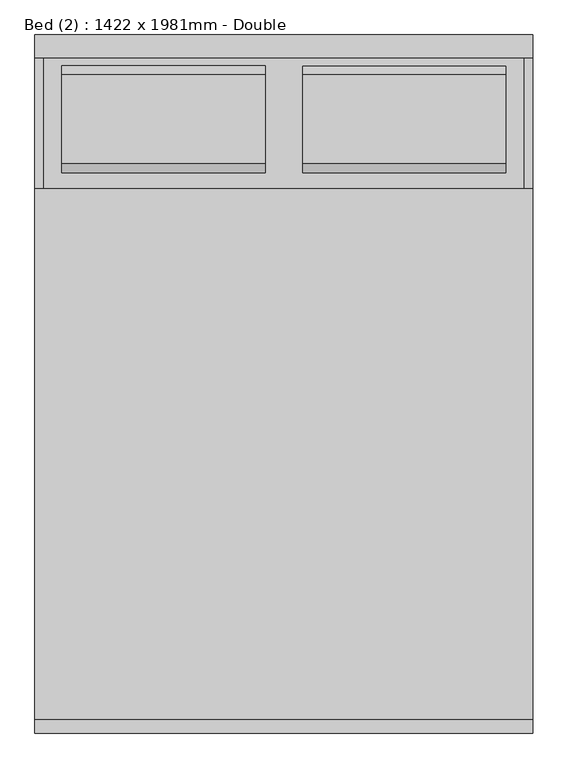
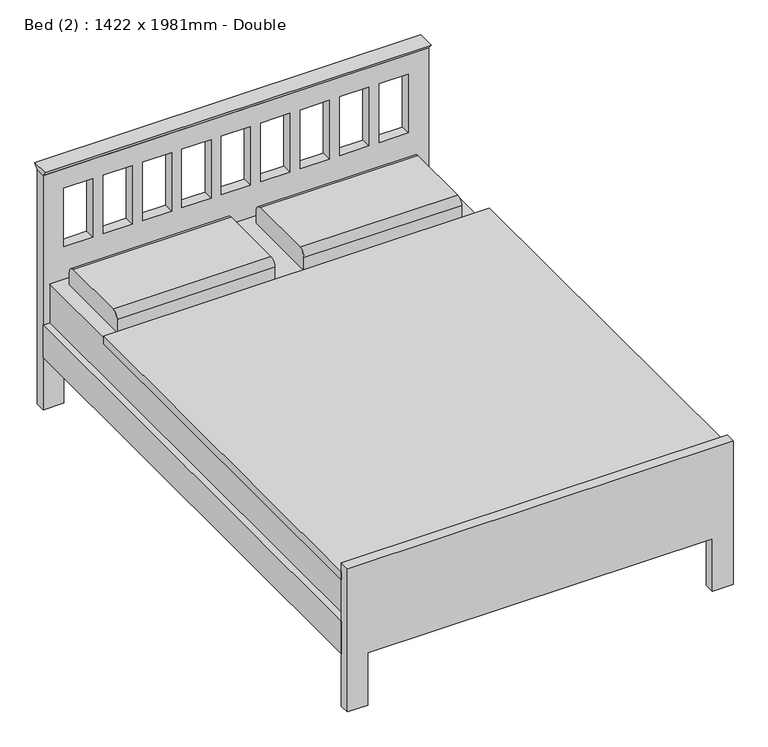
"""IFC4 building model written with IfcOpenShell, lengths in millimetres: furniture geometry, Bed (2) : 1422 x 1981mm - Double."""

import ifcopenshell
import ifcopenshell.guid

model = None  # the IFC model being written
_history = None  # IfcOwnerHistory: only IFC2X3 demands one
_inside = {}  # id of a spatial element -> (the spatial element, [elements in it])
_under = {}  # id of a project, library or spatial element -> (it, [spatial elements below it])
_declared = {}  # id of a project -> (the project, [libraries it declares])
_typed = {}  # id of a type object -> (the type object, [elements of that type])
_made_of = {}  # id of a material, layer set ... -> (it, [elements and type objects made of it])


def new_model(schema):
    """Start an empty IFC model of exactly this schema.

    Asked for "IFC4X3", IfcOpenShell would pick the latest addendum, in which some entities
    have other attributes; the version numbers below select the first issue.
    IFC2X3 requires an IfcOwnerHistory on every rooted entity: one is made here for all.
    """
    global model, _history
    if schema == "IFC4X3":
        model = ifcopenshell.file(schema_version=(4, 3, 0, 0))
    else:
        model = ifcopenshell.file(schema=schema)
    _inside.clear()
    _under.clear()
    _declared.clear()
    _typed.clear()
    _made_of.clear()
    _history = None
    if model.schema == "IFC2X3":
        org = make("IfcOrganization", Name="unknown")
        user = make(
            "IfcPersonAndOrganization",
            ThePerson=make("IfcPerson", FamilyName="unknown"),
            TheOrganization=org,
        )
        app = make(
            "IfcApplication",
            ApplicationDeveloper=org,
            Version="unknown",
            ApplicationFullName="unknown",
            ApplicationIdentifier="unknown",
        )
        _history = make(
            "IfcOwnerHistory",
            OwningUser=user,
            OwningApplication=app,
            ChangeAction="ADDED",
            CreationDate=0,
        )
    return model


def make(cls, **values):
    """One entity of the class cls with the attributes given. An attribute that is None is left unset."""
    return model.create_entity(
        cls, **{name: value for name, value in values.items() if value is not None}
    )


def rooted(cls, **values):
    """An entity with a GlobalId (a new one), such as an element, a storey or a relation."""
    return make(cls, GlobalId=ifcopenshell.guid.new(), OwnerHistory=_history, **values)


def si_unit(unit_type, name, prefix=None):
    """IfcSIUnit, for example si_unit("LENGTHUNIT", "METRE", prefix="MILLI")."""
    return make("IfcSIUnit", UnitType=unit_type, Prefix=prefix, Name=name)


def assignment(units):
    """IfcUnitAssignment: the units of a project."""
    return None if units is None else make("IfcUnitAssignment", Units=units)


def point(xyz):
    """IfcCartesianPoint."""
    return None if xyz is None else make("IfcCartesianPoint", Coordinates=xyz)


def direction(xyz):
    """IfcDirection."""
    return None if xyz is None else make("IfcDirection", DirectionRatios=xyz)


def frame(location, z_axis=None, x_axis=None):
    """IfcAxis2Placement3D, a coordinate frame: its origin and axes. An axis left out is left unset."""
    return make(
        "IfcAxis2Placement3D",
        Location=point(location),
        Axis=direction(z_axis),
        RefDirection=direction(x_axis),
    )


def frame_2d(location, x_axis=None):
    """IfcAxis2Placement2D, a coordinate frame in the plane: its origin and x axis."""
    return make(
        "IfcAxis2Placement2D", Location=point(location), RefDirection=direction(x_axis)
    )


def origin():
    """The frame at (0, 0, 0) with its axes left unset."""
    return frame((0.0, 0.0, 0.0))


def place(relative_to, where):
    """IfcLocalPlacement: puts the frame where relative to a parent placement (None: the world)."""
    return make(
        "IfcLocalPlacement", PlacementRelTo=relative_to, RelativePlacement=where
    )


def context(
    kind, dimensions, precision=None, world=None, true_north=None, identifier=None
):
    """IfcGeometricRepresentationContext, for example the 3D "Model" context."""
    return make(
        "IfcGeometricRepresentationContext",
        ContextIdentifier=identifier,
        ContextType=kind,
        CoordinateSpaceDimension=dimensions,
        Precision=precision,
        WorldCoordinateSystem=world,
        TrueNorth=true_north,
    )


def project(units=None, contexts=None):
    """IfcProject with its units and contexts."""
    return rooted(
        "IfcProject",
        Name="project",
        RepresentationContexts=contexts,
        UnitsInContext=assignment(units),
    )


def spatial(cls, under=None, at=None, **own):
    """A site, building, storey or space (cls), placed at a placement, below another one or the project."""
    s = rooted(cls, ObjectPlacement=at, **own)
    if under is not None:
        _under.setdefault(under.id(), (under, []))[1].append(s)
    return s


def polyline(points):
    """IfcPolyline through the points."""
    return make("IfcPolyline", Points=[point(p) for p in points])


def circle_curve(where, radius):
    """IfcCircle in the frame where."""
    return make("IfcCircle", Position=where, Radius=radius)


def trimmed(basis, trim1, trim2, sense, master):
    """IfcTrimmedCurve: the piece of a basis curve between two trims."""
    return make(
        "IfcTrimmedCurve",
        BasisCurve=basis,
        Trim1=trim1,
        Trim2=trim2,
        SenseAgreement=sense,
        MasterRepresentation=master,
    )


def segment(curve, same_sense, transition):
    """IfcCompositeCurveSegment."""
    return make(
        "IfcCompositeCurveSegment",
        Transition=transition,
        SameSense=same_sense,
        ParentCurve=curve,
    )


def composite_curve(segments, self_intersect=None):
    """IfcCompositeCurve: segments joined end to end."""
    return make("IfcCompositeCurve", Segments=segments, SelfIntersect=self_intersect)


def outline(outer, holes=None, kind="AREA"):
    """IfcArbitraryClosedProfileDef: a profile drawn as a closed curve; with holes, ...WithVoids."""
    if holes is None:
        return make("IfcArbitraryClosedProfileDef", ProfileType=kind, OuterCurve=outer)
    return make(
        "IfcArbitraryProfileDefWithVoids",
        ProfileType=kind,
        OuterCurve=outer,
        InnerCurves=holes,
    )


def extrude(swept, where, along, depth):
    """IfcExtrudedAreaSolid: the profile swept, set in the frame where, extruded along a direction by depth."""
    return make(
        "IfcExtrudedAreaSolid",
        SweptArea=swept,
        Position=where,
        ExtrudedDirection=direction(along),
        Depth=depth,
    )


def shape(context_of_items, identifier, shape_type, items):
    """IfcShapeRepresentation: the items that make up one representation, for example the "Body"."""
    return make(
        "IfcShapeRepresentation",
        ContextOfItems=context_of_items,
        RepresentationIdentifier=identifier,
        RepresentationType=shape_type,
        Items=items,
    )


def source(mapping_origin, context_of_items, identifier, shape_type, items):
    """IfcRepresentationMap: a shape defined once, which mapped items show again and again."""
    return make(
        "IfcRepresentationMap",
        MappingOrigin=mapping_origin,
        MappedRepresentation=shape(context_of_items, identifier, shape_type, items),
    )


def transform(
    local_origin,
    x_axis=None,
    y_axis=None,
    z_axis=None,
    scale=None,
    scale2=None,
    scale3=None,
    uniform=True,
):
    """IfcCartesianTransformationOperator3D, or its non-uniform kind. x_axis, y_axis, z_axis: its Axis1, 2, 3."""
    if uniform:
        return make(
            "IfcCartesianTransformationOperator3D",
            Axis1=direction(x_axis),
            Axis2=direction(y_axis),
            LocalOrigin=point(local_origin),
            Scale=scale,
            Axis3=direction(z_axis),
        )
    return make(
        "IfcCartesianTransformationOperator3DnonUniform",
        Axis1=direction(x_axis),
        Axis2=direction(y_axis),
        LocalOrigin=point(local_origin),
        Scale=scale,
        Axis3=direction(z_axis),
        Scale2=scale2,
        Scale3=scale3,
    )


def mapped(mapping_source, mapping_target):
    """IfcMappedItem: shows the shape of a source again, moved by a transform."""
    return make(
        "IfcMappedItem", MappingSource=mapping_source, MappingTarget=mapping_target
    )


def made_of(thing, what):
    """Note that an element or type object is made of a material, layer set ...; save() writes the relation."""
    if what is not None:
        _made_of.setdefault(what.id(), (what, []))[1].append(thing)
    return thing


def element(
    cls,
    number,
    at=None,
    inside=None,
    cuts=None,
    type_object=None,
    material=None,
    context=None,
    identifier="Body",
    shape_type=None,
    held_by="IfcProductDefinitionShape",
    body=None,
    shapes=None,
    **own,
):
    """One element of the class cls, such as IfcWall. Its Tag is "e" and its number.

    at: its placement. inside: the storey or other place that contains it. cuts: it is an
    opening in that element (IfcRelVoidsElement). A single representation is given by context,
    identifier, shape_type and body (its items); several are given by shapes. held_by: the class
    of the entity that holds the representations. save() writes the other relations.
    """
    e = rooted(cls, Tag="e%d" % number, ObjectPlacement=at, **own)
    if body is not None:
        shapes = [shape(context, identifier, shape_type, body)]
    if shapes is not None:
        e.Representation = make(held_by, Representations=shapes)
    if inside is not None:
        _inside.setdefault(inside.id(), (inside, []))[1].append(e)
    if cuts is not None:
        rooted(
            "IfcRelVoidsElement", RelatingBuildingElement=cuts, RelatedOpeningElement=e
        )
    if type_object is not None:
        _typed.setdefault(type_object.id(), (type_object, []))[1].append(e)
    return made_of(e, material)


def aggregate(whole, parts):
    """IfcRelAggregates: a whole, such as a stair, and the parts it consists of."""
    return rooted("IfcRelAggregates", RelatingObject=whole, RelatedObjects=parts)


def save(model, path):
    """Write the relations noted so far, then the file.

    IfcRelAggregates (storeys below a building ...), IfcRelContainedInSpatialStructure (elements
    in a storey), IfcRelDefinesByType, IfcRelAssociatesMaterial and IfcRelDeclares: one each for
    every whole, place, type object, material and project.
    """
    for whole, parts in _under.values():
        aggregate(whole, parts)
    for where, things in _inside.values():
        rooted(
            "IfcRelContainedInSpatialStructure",
            RelatedElements=things,
            RelatingStructure=where,
        )
    for kind, things in _typed.values():
        rooted("IfcRelDefinesByType", RelatedObjects=things, RelatingType=kind)
    for what, things in _made_of.values():
        rooted("IfcRelAssociatesMaterial", RelatedObjects=things, RelatingMaterial=what)
    for by, libraries in _declared.values():
        rooted("IfcRelDeclares", RelatingContext=by, RelatedDefinitions=libraries)
    model.write(path)


def bed_2_1422_x_1981mm_double_43666e8e(model_context):
    return source(origin(), model_context, "Body", "SweptSolid", [
        extrude(outline(composite_curve([segment(polyline([(-380.0, 482.55), (-380.0, 533.35)]), True, "CONTINUOUS"), segment(trimmed(circle_curve(frame_2d((-354.6, 533.35)), 25.4), [point((-380.0, 533.35))], [point((-354.6, 558.75))], False, "CARTESIAN"), True, "CONTINUOUS"), segment(polyline([(-354.6, 558.75), (-100.6, 558.75)]), True, "CONTINUOUS"), segment(trimmed(circle_curve(frame_2d((-100.6, 533.35)), 25.4), [point((-100.6, 558.75))], [point((-75.2, 533.35))], False, "CARTESIAN"), True, "CONTINUOUS"), segment(polyline([(-75.2, 533.35), (-75.2, 482.55), (-380.0, 482.55)]), True, "CONTINUOUS")], self_intersect=False)), frame((34.5722222, 0.0, 0.0), z_axis=(1.0, 0.0, 0.0), x_axis=(0.0, 1.0, 0.0)), (0.0, 0.0, 1.0), 581.3777778),
        extrude(outline(polyline([(-38.1, 914.4), (-51.9545455, 933.45), (13.8545455, 933.45), (0.0, 914.4), (-38.1, 914.4)])), frame((-730.0365546, 0.0, 0.0), z_axis=(1.0, 0.0, 0.0), x_axis=(0.0, 1.0, 0.0)), (0.0, 0.0, 1.0), 1422.4533613),
        extrude(outline(composite_curve([segment(polyline([(-379.4173224, 482.6), (-379.4173224, 533.4)]), True, "CONTINUOUS"), segment(trimmed(circle_curve(frame_2d((-354.0173224, 533.4)), 25.4), [point((-379.4173224, 533.4))], [point((-354.0173224, 558.8))], False, "CARTESIAN"), True, "CONTINUOUS"), segment(polyline([(-354.0173224, 558.8), (-100.0173224, 558.8)]), True, "CONTINUOUS"), segment(trimmed(circle_curve(frame_2d((-100.0173224, 533.4)), 25.4), [point((-100.0173224, 558.8))], [point((-74.6173224, 533.4))], False, "CARTESIAN"), True, "CONTINUOUS"), segment(polyline([(-74.6173224, 533.4), (-74.6173224, 482.6), (-379.4173224, 482.6)]), True, "CONTINUOUS")], self_intersect=False)), frame((-654.05, 0.0, 0.0), z_axis=(1.0, 0.0, 0.0), x_axis=(0.0, 1.0, 0.0)), (0.0, 0.0, 1.0), 581.3777778),
        extrude(outline(polyline([(666.75, -38.1), (666.75, -1943.1), (-704.85, -1943.1), (-704.85, -38.1), (666.75, -38.1)])), frame((0.0, 0.0, 203.2), z_axis=(0.0, 0.0, 1.0), x_axis=(1.0, 0.0, 0.0)), (0.0, 0.0, 1.0), 279.4),
        extrude(outline(polyline([(666.75, -1943.1), (666.75, -38.1), (692.15, -38.1), (692.15, -1943.1), (666.75, -1943.1)])), frame((0.0, 0.0, 203.0994861), z_axis=(0.0, 0.0, 1.0), x_axis=(1.0, 0.0, 0.0)), (0.0, 0.0, 1.0), 127.0),
        extrude(outline(polyline([(-730.25, -1943.1), (-730.25, -38.1), (-704.85, -38.1), (-704.85, -1943.1), (-730.25, -1943.1)])), frame((0.0, 0.0, 203.5755296), z_axis=(0.0, 0.0, 1.0), x_axis=(1.0, 0.0, 0.0)), (0.0, 0.0, 1.0), 127.0),
        extrude(outline(polyline([(0.0, -654.05), (203.2, -654.05), (203.2, 615.95), (0.0, 615.95), (0.0, 692.15), (558.8, 692.15), (558.8, -730.25), (0.0, -730.25), (0.0, -654.05)])), frame((0.0, -1981.2, 0.0), z_axis=(0.0, 1.0, 0.0), x_axis=(0.0, 0.0, 1.0)), (0.0, 0.0, 1.0), 38.1),
        extrude(outline(polyline([(914.4, 692.4168067), (914.4, -730.0365546), (0.0, -730.0365546), (0.0, -654.05), (203.2, -654.05), (203.2, 615.95), (0.0, 615.95), (0.0, 692.4168067), (914.4, 692.4168067)]), holes=[polyline([(838.2, -546.8055556), (609.6, -546.8055556), (609.6, -654.05), (838.2, -654.05), (838.2, -546.8055556)]), polyline([(838.2, -401.4611111), (609.6, -401.4611111), (609.6, -508.7055556), (838.2, -508.7055556), (838.2, -401.4611111)]), polyline([(838.2, -256.1166667), (609.6, -256.1166667), (609.6, -363.3611111), (838.2, -363.3611111), (838.2, -256.1166667)]), polyline([(838.2, -110.7722222), (609.6, -110.7722222), (609.6, -218.0166667), (838.2, -218.0166667), (838.2, -110.7722222)]), polyline([(838.2, 179.9166667), (609.6, 179.9166667), (609.6, 72.6722222), (838.2, 72.6722222), (838.2, 179.9166667)]), polyline([(838.2, 325.2611111), (609.6, 325.2611111), (609.6, 218.0166667), (838.2, 218.0166667), (838.2, 325.2611111)]), polyline([(838.2, 470.6055556), (609.6, 470.6055556), (609.6, 363.3611111), (838.2, 363.3611111), (838.2, 470.6055556)]), polyline([(838.2, 615.95), (609.6, 615.95), (609.6, 508.7055556), (838.2, 508.7055556), (838.2, 615.95)]), polyline([(838.2, 34.5722222), (609.6, 34.5722222), (609.6, -72.6722222), (838.2, -72.6722222), (838.2, 34.5722222)])]), frame((0.0, -38.1, 0.0), z_axis=(0.0, 1.0, 0.0), x_axis=(0.0, 0.0, 1.0)), (0.0, 0.0, 1.0), 38.1),
        extrude(outline(polyline([(-730.25, -1943.1), (-730.25, -425.390138), (692.15, -425.390138), (692.15, -1943.1), (-730.25, -1943.1)])), frame((0.0, 0.0, 492.6), z_axis=(0.0, 0.0, 1.0), x_axis=(1.0, 0.0, 0.0)), (0.0, 0.0, 1.0), 31.2),
    ])


if __name__ == "__main__":
    model = new_model("IFC4")
    model_context = context("Model", 3, world=origin())
    ifc_project = project(units=[si_unit("LENGTHUNIT", "METRE", prefix="MILLI")], contexts=[model_context])
    site = spatial("IfcSite", under=ifc_project)
    building = spatial("IfcBuilding", under=site)
    placement = place(None, origin())
    bed_2_1422_x_1981mm_double_shape = bed_2_1422_x_1981mm_double_43666e8e(model_context)
    element("IfcFurniture", 1, ObjectType="Bed (2) : 1422 x 1981mm - Double", at=placement, inside=building, context=model_context, shape_type="MappedRepresentation", body=[
        mapped(bed_2_1422_x_1981mm_double_shape, transform((0.0, 0.0, 0.0), x_axis=(1.0, 0.0, 0.0), y_axis=(0.0, 1.0, 0.0), z_axis=(0.0, 0.0, 1.0))),
    ])
    save(model, "model.ifc")

# Revit data of these elements
# Project information
#   Document_Suitability_Code = "S01"
#   Document_Suitability_Description = "Coordination"
#   Project Status = "Project Status"
#   Client Name = "Revit Project"
#   Project Address = "Enter address here"
#   Project Name = "Two Storey Residence"
#   Project Number = "RARC01"
# Type "Bed (2) : 1422 x 1981mm - Double"
#   Keynote = "N"
#   Length = 1981.2 mm
#   Width = 1422.4 mm
#   Material Frame = Wood - Birch
#   Material Mattress = Textile - White
#   Default Elevation = 0
# Element 1 (IfcFurniture, "Bed (2) : 1422 x 1981mm - Double")
#   Materials on its faces: "Wood - Birch", "Textile - White"
# Materials
#   "Wood - Birch": class "Wood", colour RGB 224 178 126, transparency 0
#   "Textile - White": class "Fabric", colour RGB 247 247 239, transparency 0
